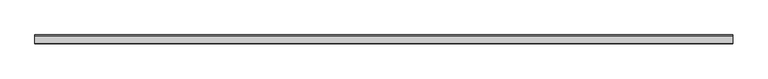
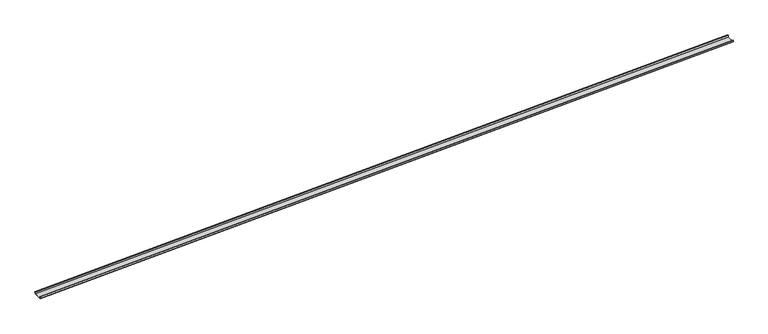
"""IFC4 building model written with IfcOpenShell, lengths in millimetres: proxy geometry, Generic Models 2:Generic Models 2:310765:Generic Models 2:310765 : Generic Models 2:Generic Models 2:310765:147 : Generic Models 2:Generic Models 2:310765:Generic Models 2:310765 : Generic Models 2:Generic Models 2:310765:300385."""

from ifc_helpers import new_model, si_unit, frame, origin, place, context, project, spatial, polyline, outline, extrude, source, transform, mapped, element, save


def generic_models_ca6124e0(model_context):
    return source(origin(), model_context, "Body", "SweptSolid", [
        extrude(outline(polyline([(1.5875, 0.0), (1.5875, 50.8), (223.8375, 50.8), (223.8375, 1.5874999), (222.25, 1.5874999), (222.25, 49.2124999), (3.175, 49.2124999), (3.175, -1.5875), (-14.2875, -1.5875), (-14.2875, 9.525), (-12.7, 9.525), (-12.7, 0.0), (1.5875, 0.0)])), frame((560326.4711757, -578522.5893007, 3999.10949), z_axis=(0.9991330730923568, 0.0, 0.041630544712067834), x_axis=(0.0, -1.0, 0.0)), (0.0, 0.0, 1.0), 18740.1587223),
    ])


if __name__ == "__main__":
    model = new_model("IFC4")
    model_context = context("Model", 3, world=origin())
    ifc_project = project(units=[si_unit("LENGTHUNIT", "METRE", prefix="MILLI")], contexts=[model_context])
    site = spatial("IfcSite", under=ifc_project)
    building = spatial("IfcBuilding", under=site)
    placement = place(None, origin())
    generic_models_shape = generic_models_ca6124e0(model_context)
    element("IfcBuildingElementProxy", 1, Name="Generic Models 2:Generic Models 2:310765:Generic Models 2:310765 : Generic Models 2:Generic Models 2:310765:147 : Generic Models 2:Generic Models 2:310765:Generic Models 2:310765 : Generic Models 2:Generic Models 2:310765:300385", ObjectType="Generic Models 2:Generic Models 2:310765:Generic Models 2:310765 : Generic Models 2:Generic Models 2:310765:147 : Generic Models 2:Generic Models 2:310765:Generic Models 2:310765 : Generic Models 2:Generic Models 2:310765:300385", at=placement, inside=building, context=model_context, shape_type="MappedRepresentation", body=[
        mapped(generic_models_shape, transform((0.0, 0.0, 0.0), x_axis=(1.0, 0.0, 0.0), y_axis=(0.0, 1.0, 0.0), z_axis=(0.0, 0.0, 1.0))),
    ])
    save(model, "model.ifc")

# Revit data of these elements
# Type "Generic Models 2:Generic Models 2:310765:Generic Models 2:310765 : Generic Models 2:Generic Models 2:310765:147 : Generic Models 2:Generic Models 2:310765:Generic Models 2:310765 : Generic Models 2:Generic Models 2:310765:300385"
#   NameOverride = "Generic Models 2:Generic Models 2:310765:Generic Models 2:310765 : Generic Models 2:Generic Models 2:310765:300385"
#   ObjectTypeOverride = "Generic Models 2:310765 : Generic Models 2:Generic Models 2:310765"
#   Reference = "Generic Models 2"
#   Tag = "300385"
# Element 1 (IfcBuildingElementProxy, "Generic Models 2:Generic Models 2:310765:Generic Models 2:310765 : Generic Models 2:Generic Models 2:310765:147 : Generic Models 2:Generic Models 2:310765:Generic Models 2:310765 : Generic Models 2:Generic Models 2:310765:300385")
#   Materials on its faces: "STRUCTURAL STANDING SEAM SHEET METAL ROOFING - BATTENLOK - COLOR T.B.D."
# Materials
#   "STRUCTURAL STANDING SEAM SHEET METAL ROOFING - BATTENLOK - COLOR T.B.D.": class "Generic", colour RGB 120 120 120, transparency 0, Cost = 0
